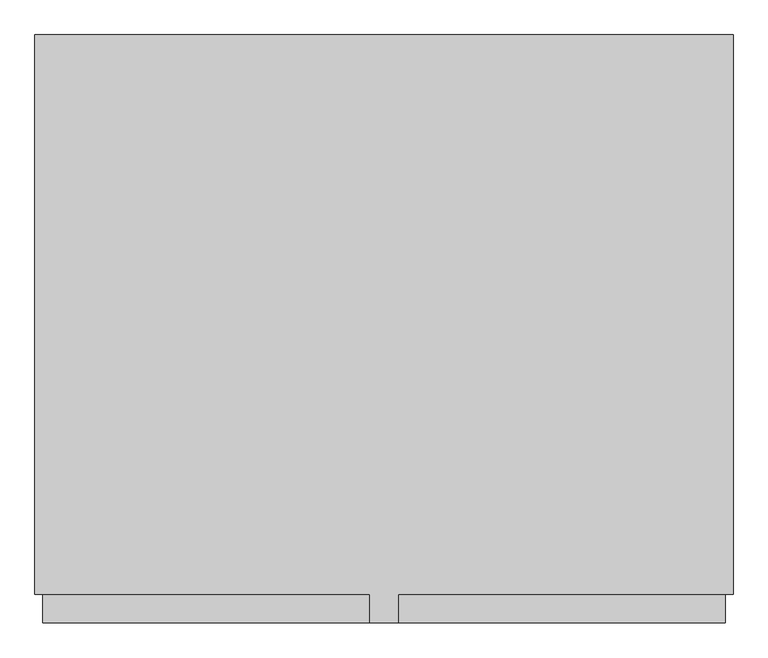
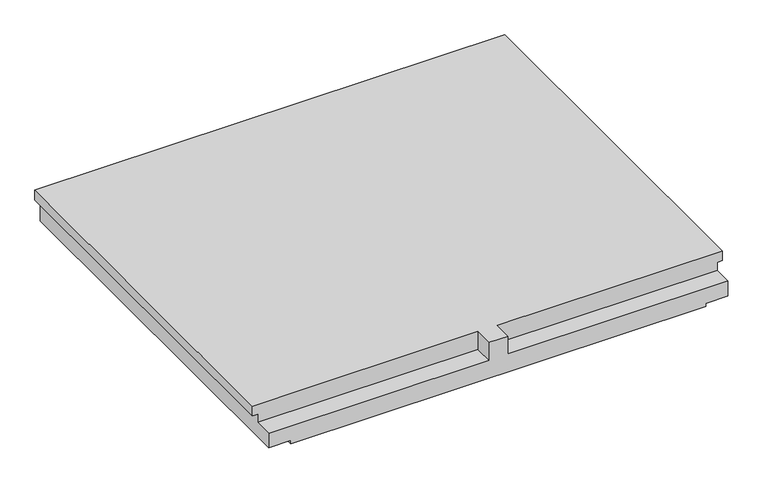
"""IFC4 building model written with IfcOpenShell, lengths in millimetres: proxy geometry, NLRS_24_GM_UN_rechthoekig bordes prefab-AV_gen_rsf : prefab bordes_gen__2300x2730."""

from ifc_helpers import new_model, si_unit, origin, place, context, project, spatial, faceted_brep, source, transform, mapped, element, save


def generic_models_c7907445(model_context):
    return source(origin(), model_context, "Body", "Brep", [
        faceted_brep([(1365.0, -2190.0, 0.0), (1365.0, -2190.0, -60.0), (1365.0, 0.0, -60.0), (1365.0, 0.0, 0.0), (55.0, -2300.0, -110.0), (1335.0, -2300.0, -110.0), (1335.0, -2190.0, -110.0), (55.0, -2190.0, -110.0), (55.0, -2190.0, 0.0), (1335.0, -2190.0, -60.0), (55.0, -2300.0, 0.0), (-55.0, -2300.0, 0.0), (-55.0, -2190.0, 0.0), (-55.0, -2190.0, -110.0), (-55.0, -2300.0, -110.0), (-1365.0, 0.0, 0.0), (-1365.0, 0.0, -60.0), (-1365.0, -2190.0, -60.0), (-1365.0, -2190.0, 0.0), (-1335.0, -2300.0, -110.0), (-1335.0, -2300.0, -200.0), (-1205.0, -2300.0, -200.0), (-1205.0, -2300.0, -220.0), (1205.0, -2300.0, -220.0), (1205.0, -2300.0, -200.0), (1335.0, -2300.0, -200.0), (-1335.0, -2190.0, -110.0), (-1335.0, -2190.0, -60.0), (1335.0, 0.0, -60.0), (1335.0, 0.0, -200.0), (1205.0, 0.0, -200.0), (1205.0, 0.0, -220.0), (-1205.0, 0.0, -220.0), (-1205.0, 0.0, -200.0), (-1335.0, 0.0, -200.0), (-1335.0, 0.0, -60.0)], [[[0, 1, 2, 3]], [[4, 5, 6, 7]], [[8, 7, 6, 9, 1, 0]], [[10, 4, 7, 8]], [[11, 12, 13, 14]], [[15, 16, 17, 18]], [[19, 20, 21, 22, 23, 24, 25, 5, 4, 10, 11, 14]], [[14, 13, 26, 19]], [[18, 17, 27, 26, 13, 12]], [[18, 12, 11, 10, 8, 0, 3, 15]], [[15, 3, 2, 28, 29, 30, 31, 32, 33, 34, 35, 16]], [[32, 31, 23, 22]], [[27, 17, 16, 35]], [[20, 19, 26, 27, 35, 34]], [[34, 33, 21, 20]], [[33, 32, 22, 21]], [[28, 2, 1, 9]], [[29, 28, 9, 6, 5, 25]], [[25, 24, 30, 29]], [[24, 23, 31, 30]]]),
    ])


if __name__ == "__main__":
    model = new_model("IFC4")
    model_context = context("Model", 3, world=origin())
    ifc_project = project(units=[si_unit("LENGTHUNIT", "METRE", prefix="MILLI")], contexts=[model_context])
    site = spatial("IfcSite", under=ifc_project)
    building = spatial("IfcBuilding", under=site)
    placement = place(None, origin())
    generic_models_shape = generic_models_c7907445(model_context)
    element("IfcBuildingElementProxy", 1, Name="NLRS_24_GM_UN_rechthoekig bordes prefab-AV_gen_rsf : prefab bordes_gen__2300x2730", ObjectType="NLRS_24_GM_UN_rechthoekig bordes prefab-AV_gen_rsf : prefab bordes_gen__2300x2730", at=placement, inside=building, context=model_context, shape_type="MappedRepresentation", body=[
        mapped(generic_models_shape, transform((0.0, 0.0, 0.0), x_axis=(1.0, 0.0, 0.0), y_axis=(0.0, 1.0, 0.0), z_axis=(0.0, 0.0, 1.0))),
    ])
    save(model, "model.ifc")

# Revit data of these elements
# Type "NLRS_24_GM_UN_rechthoekig bordes prefab-AV_gen_rsf : prefab bordes_gen__2300x2730"
#   Export Type to IFC As = "IfcStair"
#   Type IfcGUID = "2CEqVLPNH8KRN7ghwV3ZdG"
#   Type Comments = " "
#   Model = " "
#   Manufacturer = " "
#   Description = "rechthoekig bordes prefab\r\n1930x4395"
#   Assembly Code = "24.15"
#   Width = 2730 mm
#   Thickness = 220 mm
#   Perimeter = 10060 mm
#   NLRS_C_lengte_02 = 1310 mm
#   NLRS_C_lengte_01 = 1310 mm
#   NLRS_C_hoogte_02 = 110 mm
#   NLRS_C_hoogte_01 = 110 mm
#   NLRS_C_diepte_04 = 2300 mm
#   NLRS_C_diepte_03 = 2300 mm
#   NLRS_C_diepte_02 = 110 mm
#   NLRS_C_diepte_01 = 110 mm
#   Length = 2300 mm
#   Default Elevation = 1219.2 mm
#   Area = 6.279 m²
#   NLRS_C_materiaal = NLRS_f2_beton prefab_gen_rsf
#   Keynote = ""
# Element 1 (IfcBuildingElementProxy, "NLRS_24_GM_UN_rechthoekig bordes prefab-AV_gen_rsf : prefab bordes_gen__2300x2730")
#   Materials on its faces: "NLRS_f2_beton prefab_gen_rsf"
# Materials
#   "NLRS_f2_beton prefab_gen_rsf": class "F - Niet gebakken kunststeen", colour RGB 129 133 118, transparency 0, Keynote = "f2", Manufacturer = "Revit Standards Foundation", URL = "www.revitstandards.org", Description = "beton prefab", Cost = 0
